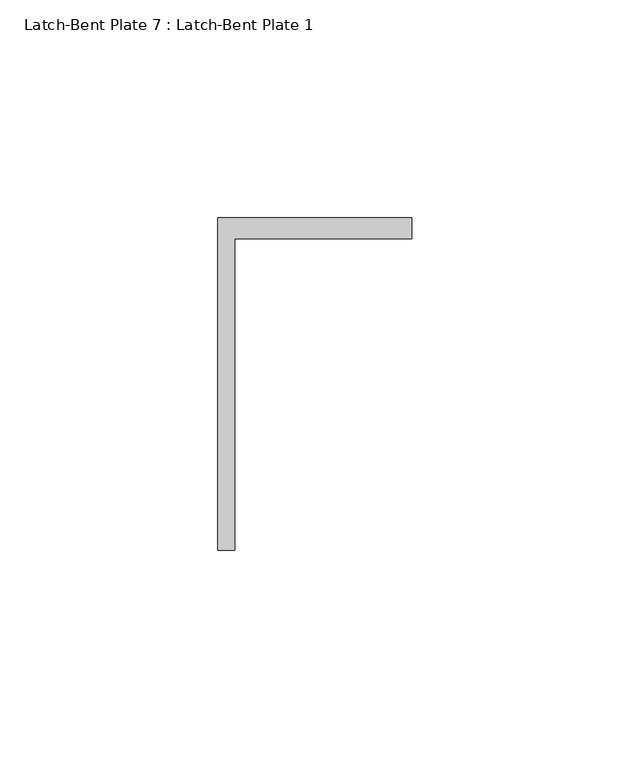
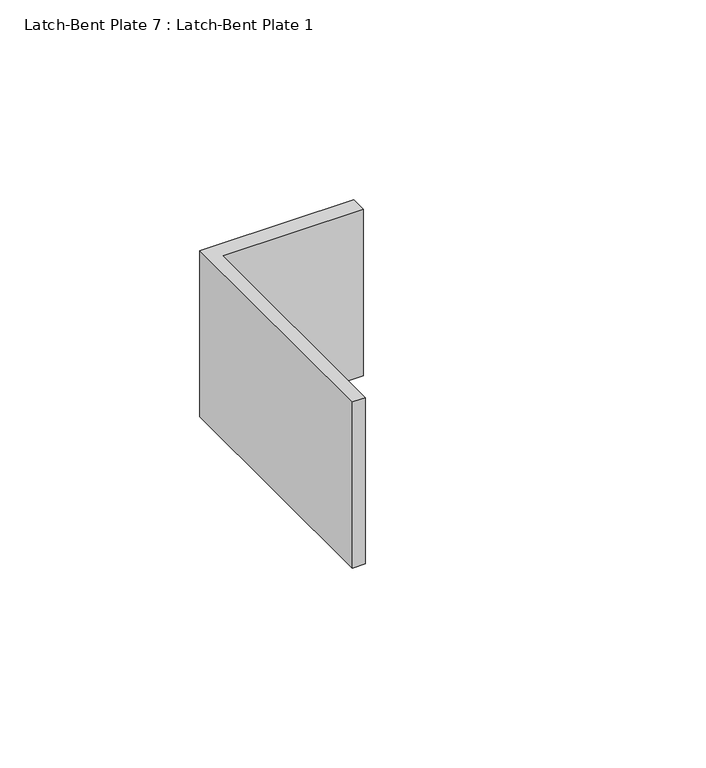
"""IFC4 building model written with IfcOpenShell, lengths in millimetres: proxy geometry, Latch-Bent Plate 7 : Latch-Bent Plate 1."""

from ifc_helpers import new_model, si_unit, frame, origin, place, context, project, spatial, polyline, outline, extrude, source, transform, mapped, element, save


def latch_bent_plate_7_latch_bent_plate_1_70bb7140(model_context):
    return source(origin(), model_context, "Body", "SweptSolid", [
        extrude(outline(polyline([(587327.0060739, -535207.9163841), (587366.6808739, -535207.9163841), (587366.6808739, -535212.6788841), (587326.1141748, -535212.6788841), (587326.1141748, -535284.1163841), (587322.2435739, -535284.1163841), (587322.2435739, -535207.9163841), (587327.0060739, -535207.9163841)])), frame((0.0, 0.0, 1041.4), z_axis=(0.0, 0.0, 1.0), x_axis=(1.0, 0.0, 0.0)), (0.0, 0.0, 1.0), 50.8),
    ])


if __name__ == "__main__":
    model = new_model("IFC4")
    model_context = context("Model", 3, world=origin())
    ifc_project = project(units=[si_unit("LENGTHUNIT", "METRE", prefix="MILLI")], contexts=[model_context])
    site = spatial("IfcSite", under=ifc_project)
    building = spatial("IfcBuilding", under=site)
    placement = place(None, origin())
    latch_bent_plate_7_latch_bent_plate_1_shape = latch_bent_plate_7_latch_bent_plate_1_70bb7140(model_context)
    element("IfcBuildingElementProxy", 1, Name="Latch-Bent Plate 7 : Latch-Bent Plate 1", ObjectType="Latch-Bent Plate 7 : Latch-Bent Plate 1", at=placement, inside=building, context=model_context, shape_type="MappedRepresentation", body=[
        mapped(latch_bent_plate_7_latch_bent_plate_1_shape, transform((0.0, 0.0, 0.0), x_axis=(1.0, 0.0, 0.0), y_axis=(0.0, 1.0, 0.0), z_axis=(0.0, 0.0, 1.0))),
    ])
    save(model, "model.ifc")

# Revit data of these elements
# Element 1 (IfcBuildingElementProxy, "Latch-Bent Plate 7 : Latch-Bent Plate 1")
#   Materials on its faces: "GALV. GATE LATCH"
# Materials
#   "GALV. GATE LATCH": class "Metal", colour RGB 189 187 185, transparency 0, Description = "Carbon steel", Cost = 0
